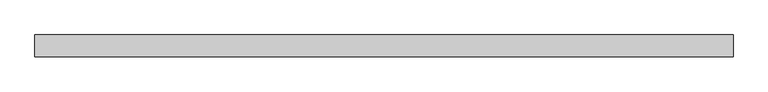
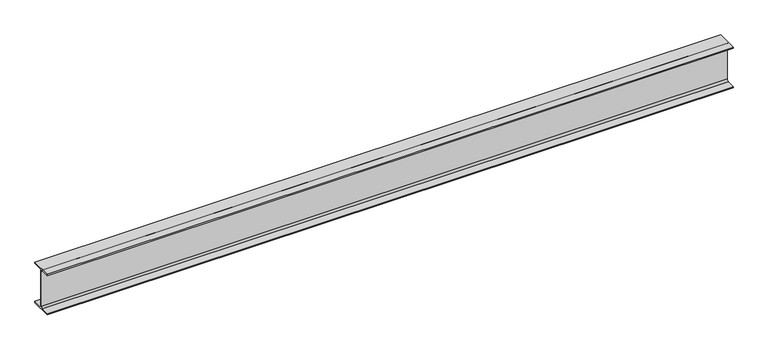
"""IFC4 building model written with IfcOpenShell, lengths in millimetres: beam geometry, 0912_Steel Framing_H-KSD3502 : H_SB_AR_S02_H-300x150x6.5x9_Stair."""

from ifc_helpers import new_model, si_unit, point, frame, frame_2d, origin, place, context, project, spatial, polyline, circle_curve, trimmed, segment, composite_curve, outline, extrude, source, transform, mapped, element, save


def beam_c00964ff(model_context):
    return source(origin(), model_context, "Body", "SweptSolid", [
        extrude(outline(composite_curve([segment(polyline([(75.0, -141.0), (75.0, -150.0), (-75.0, -150.0), (-75.0, -141.0), (-16.25, -141.0)]), True, "CONTINUOUS"), segment(trimmed(circle_curve(frame_2d((-16.25, -128.0)), 13.0), [point((-16.25, -141.0))], [point((-3.25, -128.0))], True, "CARTESIAN"), True, "CONTINUOUS"), segment(polyline([(-3.25, -128.0), (-3.25, 128.0)]), True, "CONTINUOUS"), segment(trimmed(circle_curve(frame_2d((-16.25, 128.0)), 13.0), [point((-3.25, 128.0))], [point((-16.25, 141.0))], True, "CARTESIAN"), True, "CONTINUOUS"), segment(polyline([(-16.25, 141.0), (-75.0, 141.0), (-75.0, 150.0), (75.0, 150.0), (75.0, 141.0), (16.25, 141.0)]), True, "CONTINUOUS"), segment(trimmed(circle_curve(frame_2d((16.25, 128.0)), 13.0), [point((16.25, 141.0))], [point((3.25, 128.0))], True, "CARTESIAN"), True, "CONTINUOUS"), segment(polyline([(3.25, 128.0), (3.25, -128.0)]), True, "CONTINUOUS"), segment(trimmed(circle_curve(frame_2d((16.25, -128.0)), 13.0), [point((3.25, -128.0))], [point((16.25, -141.0))], True, "CARTESIAN"), True, "CONTINUOUS"), segment(polyline([(16.25, -141.0), (75.0, -141.0)]), True, "CONTINUOUS")], self_intersect=False)), frame((-2399.8, 0.0, 0.0), z_axis=(1.0, 0.0, 0.0), x_axis=(0.0, 1.0, 0.0)), (0.0, 0.0, 1.0), 4799.6),
    ])


if __name__ == "__main__":
    model = new_model("IFC4")
    model_context = context("Model", 3, world=origin())
    ifc_project = project(units=[si_unit("LENGTHUNIT", "METRE", prefix="MILLI")], contexts=[model_context])
    site = spatial("IfcSite", under=ifc_project)
    building = spatial("IfcBuilding", under=site)
    placement = place(None, origin())
    beam_shape = beam_c00964ff(model_context)
    element("IfcBeam", 1, ObjectType="0912_Steel Framing_H-KSD3502 : H_SB_AR_S02_H-300x150x6.5x9_Stair", at=placement, inside=building, context=model_context, shape_type="MappedRepresentation", body=[
        mapped(beam_shape, transform((0.0, 0.0, 0.0), x_axis=(1.0, 0.0, 0.0), y_axis=(0.0, 1.0, 0.0), z_axis=(0.0, 0.0, 1.0))),
    ])
    save(model, "model.ifc")

# Revit data of these elements
# Type "0912_Steel Framing_H-KSD3502 : H_SB_AR_S02_H-300x150x6.5x9_Stair"
#   H_Q'ty Cal Type Tag = "SB-Q2"
#   H_WM Code_1 = "S01AA073-00001 |  | TON | Main Steel Structure Fabrication Work | Shelter/Building | Medium Steel - Standard |  |  |  |  |  |  | Material: (   ) | (90)KG/M>Weight≥(30)KG/M | S01AA073-00001 Main Steel Structure Fabrication Work Shelter/Building Medium Steel - Standard         | - Material: ( ASTM A36 )\n- (90)KG/M>Weight≥(30)KG/M"
#   H_WM Code_2 = "S03AA083-00001 |  | TON | Main Steel Structure Erection Work | Shelter/Building | Medium Steel |  |  |  |  |  |  | Material: (   ) | S03AA083-00001 Main Steel Structure Erection Work Shelter/Building Medium Steel         | - Material: ( ASTM A36 )"
#   H_WM Code_3 = "S01AA009-00001 |  | TON | Main Steel Structure Fabrication Work | Shelter/Building | Plates - Gusset, Stiffener, ETC | Material: (   ) | S01AA009-00001 Main Steel Structure Fabrication Work Shelter/Building Plates - Gusset, Stiffener, ETC         |"
#   H_WM Code_4 = "S41AA051-00001 |  | M2 | Steel Structure Paint Work | Shelter/Building | for Non-Fireproofed Steel Surface |  |  |  |  |  |  | Material: (   ) | S41AA051-00001 Steel Structure Paint Work Shelter/Building for Non-Fireproofed Steel Surface         |"
#   Width = 15.0 cm
#   Web Thickness = 0.65 cm
#   Web Fillet = 1.3 cm
#   Warping Constant = 107000.0 cm⁶
#   W = 0
#   Torsional Moment of Inertia = 9.9539 cm⁴
#   Section Area = 46.78 cm²
#   Plastic Modulus weak axis = 105.0 cm³
#   Plastic Modulus strong axis = 542.0 cm³
#   Perimeter = 1.17 m²/m
#   Nominal Weight = 36.70 kgf/m
#   Moment of Inertia weak axis = 508.00 cm⁴
#   Moment of Inertia strong axis = 7210.00 cm⁴
#   Height = 30.0 cm
#   Flange Thickness = 0.9 cm
#   Elastic Modulus weak axis = 67.7 cm³
#   Elastic Modulus strong axis = 481.0 cm³
#   Centroid Vertical = 15.0 cm
#   Centroid Horizontal = 7.5 cm
#   Ix = 72100000
#   Length [instance default] = 1524 mm
#   Zx = 542000
#   b = 150 mm
#   h = 300 mm
#   r = 13 mm
#   s = 6.5 mm
#   t = 9 mm
#   A = 0.004678 m²
#   Structural Material [instance default] = Steel, 45-345
#   Assembly Code = ""
# Element 1 (IfcBeam, "0912_Steel Framing_H-KSD3502 : H_SB_AR_S02_H-300x150x6.5x9_Stair")
#   Materials on its faces: "Steel, 45-345"
# Materials
#   "Steel, 45-345": class "Metal", colour RGB 189 187 185, transparency 0, Description = "Steel 345 MPa", Cost = 0
